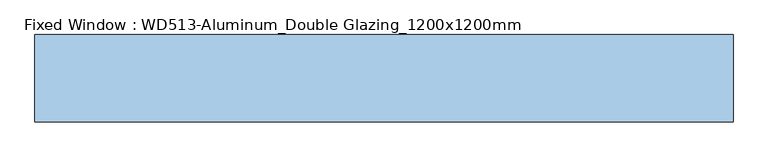
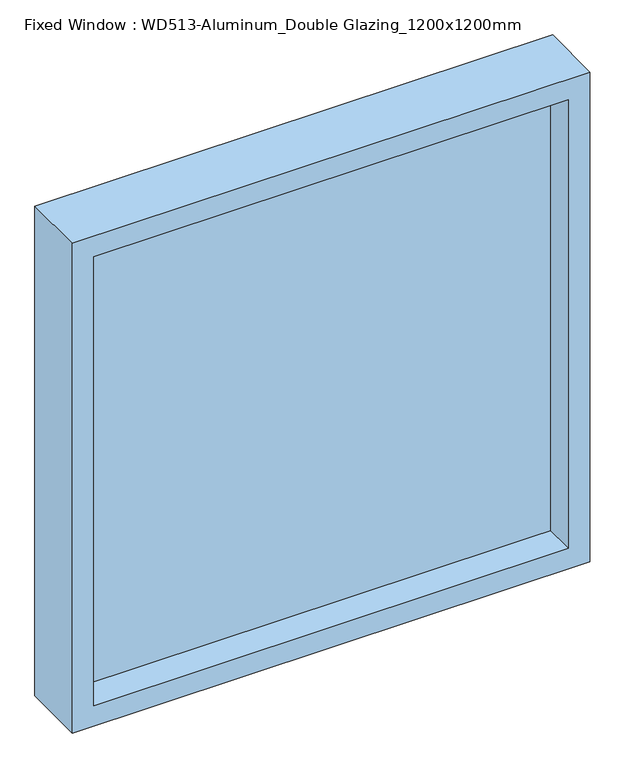
"""IFC4 building model written with IfcOpenShell, lengths in millimetres: window geometry, Fixed Window : WD513-Aluminum_Double Glazing_1200x1200mm."""

from ifc_helpers import new_model, si_unit, frame, origin, place, context, project, spatial, polyline, outline, extrude, source, transform, mapped, element, save


def fixed_window_wd513_aluminum_double_glazing_1200x1200mm_53d069df(model_context):
    return source(origin(), model_context, "Body", "SweptSolid", [
        extrude(outline(polyline([(-550.0, 3.0), (550.0, 3.0), (550.0, -3.0), (-550.0, -3.0), (-550.0, 3.0)])), frame((0.0, 0.0, 850.0), z_axis=(0.0, 0.0, 1.0), x_axis=(1.0, 0.0, 0.0)), (0.0, 0.0, 1.0), 1100.0),
        extrude(outline(polyline([(2000.0, -600.0), (800.0, -600.0), (800.0, 600.0), (2000.0, 600.0), (2000.0, -600.0)]), holes=[polyline([(1950.0, -550.0), (1950.0, 550.0), (850.0, 550.0), (850.0, -550.0), (1950.0, -550.0)])]), frame((0.0, -75.0, 0.0), z_axis=(0.0, 1.0, 0.0), x_axis=(0.0, 0.0, 1.0)), (0.0, 0.0, 1.0), 150.0),
    ])


if __name__ == "__main__":
    model = new_model("IFC4")
    model_context = context("Model", 3, world=origin())
    ifc_project = project(units=[si_unit("LENGTHUNIT", "METRE", prefix="MILLI")], contexts=[model_context])
    site = spatial("IfcSite", under=ifc_project)
    building = spatial("IfcBuilding", under=site)
    placement = place(None, origin())
    fixed_window_wd513_aluminum_double_glazing_1200x1200mm_shape = fixed_window_wd513_aluminum_double_glazing_1200x1200mm_53d069df(model_context)
    element("IfcWindow", 1, ObjectType="Fixed Window : WD513-Aluminum_Double Glazing_1200x1200mm", at=placement, inside=building, context=model_context, shape_type="MappedRepresentation", body=[
        mapped(fixed_window_wd513_aluminum_double_glazing_1200x1200mm_shape, transform((0.0, 0.0, 0.0), x_axis=(1.0, 0.0, 0.0), y_axis=(0.0, 1.0, 0.0), z_axis=(0.0, 0.0, 1.0))),
    ])
    save(model, "model.ifc")

# Revit data of these elements
# Type "Fixed Window : WD513-Aluminum_Double Glazing_1200x1200mm"
#   Description = "Aluminum Frame + 2 x T=6mm + T12mm Air Space"
#   Type Mark = ""
#   Analytic Construction = "<None>"
#   창 두께 = 150 mm
#   Height = 1200 mm
#   절반 창 두께 = 75 mm
#   기본 씰 높이 = 800 mm
#   Width = 1200 mm
#   Define Thermal Properties by = 1
#   창 패널 = AW2 창 패널
#   창 프레임 = A04AQ127-00002_Aluminum Window_None FP
#   Wall Closure = (empty or 0)
# Element 1 (IfcWindow, "Fixed Window : WD513-Aluminum_Double Glazing_1200x1200mm")
#   Materials on its faces: "A04AQ127-00002_Aluminum Window_None FP", "AW2 창 패널"
# Materials
#   "AW2 창 패널": class "유리", colour RGB 0 0 255, transparency 0.75
#   "A04AQ127-00002_Aluminum Window_None FP": class "금속", colour RGB 247 247 247, transparency 0, W00) Work Master Code = "A04AQ127-00002", W01) Work Master_Lv1 = "Finishing Work", W02) Work Master_Lv2 = "Door & Window Work", W03) Work Master_Spec.1 = "Aluminum Window", W04) Work Master_Spec.2 = "Fire Protective Rating: N/A", W05) Work Master_Spec.3 = "w/ Hardware & Accessories", Cost = 0
